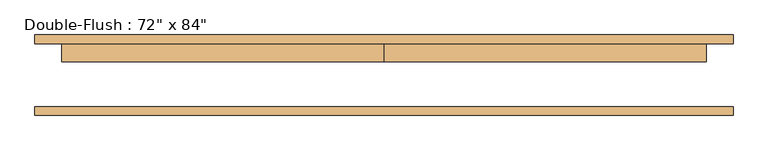
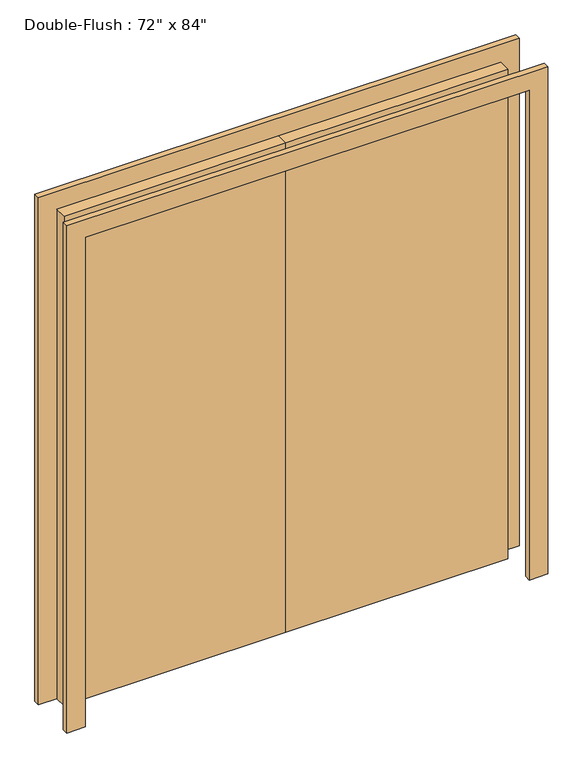
"""IFC4 building model written with IfcOpenShell, lengths in millimetres: door geometry."""

import ifcopenshell
import ifcopenshell.guid

model = None  # the IFC model being written
_history = None  # IfcOwnerHistory: only IFC2X3 demands one
_inside = {}  # id of a spatial element -> (the spatial element, [elements in it])
_under = {}  # id of a project, library or spatial element -> (it, [spatial elements below it])
_declared = {}  # id of a project -> (the project, [libraries it declares])
_typed = {}  # id of a type object -> (the type object, [elements of that type])
_made_of = {}  # id of a material, layer set ... -> (it, [elements and type objects made of it])


def new_model(schema):
    """Start an empty IFC model of exactly this schema.

    Asked for "IFC4X3", IfcOpenShell would pick the latest addendum, in which some entities
    have other attributes; the version numbers below select the first issue.
    IFC2X3 requires an IfcOwnerHistory on every rooted entity: one is made here for all.
    """
    global model, _history
    if schema == "IFC4X3":
        model = ifcopenshell.file(schema_version=(4, 3, 0, 0))
    else:
        model = ifcopenshell.file(schema=schema)
    _inside.clear()
    _under.clear()
    _declared.clear()
    _typed.clear()
    _made_of.clear()
    _history = None
    if model.schema == "IFC2X3":
        org = make("IfcOrganization", Name="unknown")
        user = make(
            "IfcPersonAndOrganization",
            ThePerson=make("IfcPerson", FamilyName="unknown"),
            TheOrganization=org,
        )
        app = make(
            "IfcApplication",
            ApplicationDeveloper=org,
            Version="unknown",
            ApplicationFullName="unknown",
            ApplicationIdentifier="unknown",
        )
        _history = make(
            "IfcOwnerHistory",
            OwningUser=user,
            OwningApplication=app,
            ChangeAction="ADDED",
            CreationDate=0,
        )
    return model


def make(cls, **values):
    """One entity of the class cls with the attributes given. An attribute that is None is left unset."""
    return model.create_entity(
        cls, **{name: value for name, value in values.items() if value is not None}
    )


def rooted(cls, **values):
    """An entity with a GlobalId (a new one), such as an element, a storey or a relation."""
    return make(cls, GlobalId=ifcopenshell.guid.new(), OwnerHistory=_history, **values)


def si_unit(unit_type, name, prefix=None):
    """IfcSIUnit, for example si_unit("LENGTHUNIT", "METRE", prefix="MILLI")."""
    return make("IfcSIUnit", UnitType=unit_type, Prefix=prefix, Name=name)


def assignment(units):
    """IfcUnitAssignment: the units of a project."""
    return None if units is None else make("IfcUnitAssignment", Units=units)


def point(xyz):
    """IfcCartesianPoint."""
    return None if xyz is None else make("IfcCartesianPoint", Coordinates=xyz)


def direction(xyz):
    """IfcDirection."""
    return None if xyz is None else make("IfcDirection", DirectionRatios=xyz)


def frame(location, z_axis=None, x_axis=None):
    """IfcAxis2Placement3D, a coordinate frame: its origin and axes. An axis left out is left unset."""
    return make(
        "IfcAxis2Placement3D",
        Location=point(location),
        Axis=direction(z_axis),
        RefDirection=direction(x_axis),
    )


def origin():
    """The frame at (0, 0, 0) with its axes left unset."""
    return frame((0.0, 0.0, 0.0))


def origin_with_axes():
    """The frame at (0, 0, 0) with the z axis (0, 0, 1) and the x axis (1, 0, 0) written out."""
    return frame((0.0, 0.0, 0.0), z_axis=(0.0, 0.0, 1.0), x_axis=(1.0, 0.0, 0.0))


def place(relative_to, where):
    """IfcLocalPlacement: puts the frame where relative to a parent placement (None: the world)."""
    return make(
        "IfcLocalPlacement", PlacementRelTo=relative_to, RelativePlacement=where
    )


def context(
    kind, dimensions, precision=None, world=None, true_north=None, identifier=None
):
    """IfcGeometricRepresentationContext, for example the 3D "Model" context."""
    return make(
        "IfcGeometricRepresentationContext",
        ContextIdentifier=identifier,
        ContextType=kind,
        CoordinateSpaceDimension=dimensions,
        Precision=precision,
        WorldCoordinateSystem=world,
        TrueNorth=true_north,
    )


def project(units=None, contexts=None):
    """IfcProject with its units and contexts."""
    return rooted(
        "IfcProject",
        Name="project",
        RepresentationContexts=contexts,
        UnitsInContext=assignment(units),
    )


def spatial(cls, under=None, at=None, **own):
    """A site, building, storey or space (cls), placed at a placement, below another one or the project."""
    s = rooted(cls, ObjectPlacement=at, **own)
    if under is not None:
        _under.setdefault(under.id(), (under, []))[1].append(s)
    return s


def polyline(points):
    """IfcPolyline through the points."""
    return make("IfcPolyline", Points=[point(p) for p in points])


def outline(outer, holes=None, kind="AREA"):
    """IfcArbitraryClosedProfileDef: a profile drawn as a closed curve; with holes, ...WithVoids."""
    if holes is None:
        return make("IfcArbitraryClosedProfileDef", ProfileType=kind, OuterCurve=outer)
    return make(
        "IfcArbitraryProfileDefWithVoids",
        ProfileType=kind,
        OuterCurve=outer,
        InnerCurves=holes,
    )


def extrude(swept, where, along, depth):
    """IfcExtrudedAreaSolid: the profile swept, set in the frame where, extruded along a direction by depth."""
    return make(
        "IfcExtrudedAreaSolid",
        SweptArea=swept,
        Position=where,
        ExtrudedDirection=direction(along),
        Depth=depth,
    )


def shape(context_of_items, identifier, shape_type, items):
    """IfcShapeRepresentation: the items that make up one representation, for example the "Body"."""
    return make(
        "IfcShapeRepresentation",
        ContextOfItems=context_of_items,
        RepresentationIdentifier=identifier,
        RepresentationType=shape_type,
        Items=items,
    )


def source(mapping_origin, context_of_items, identifier, shape_type, items):
    """IfcRepresentationMap: a shape defined once, which mapped items show again and again."""
    return make(
        "IfcRepresentationMap",
        MappingOrigin=mapping_origin,
        MappedRepresentation=shape(context_of_items, identifier, shape_type, items),
    )


def transform(
    local_origin,
    x_axis=None,
    y_axis=None,
    z_axis=None,
    scale=None,
    scale2=None,
    scale3=None,
    uniform=True,
):
    """IfcCartesianTransformationOperator3D, or its non-uniform kind. x_axis, y_axis, z_axis: its Axis1, 2, 3."""
    if uniform:
        return make(
            "IfcCartesianTransformationOperator3D",
            Axis1=direction(x_axis),
            Axis2=direction(y_axis),
            LocalOrigin=point(local_origin),
            Scale=scale,
            Axis3=direction(z_axis),
        )
    return make(
        "IfcCartesianTransformationOperator3DnonUniform",
        Axis1=direction(x_axis),
        Axis2=direction(y_axis),
        LocalOrigin=point(local_origin),
        Scale=scale,
        Axis3=direction(z_axis),
        Scale2=scale2,
        Scale3=scale3,
    )


def mapped(mapping_source, mapping_target):
    """IfcMappedItem: shows the shape of a source again, moved by a transform."""
    return make(
        "IfcMappedItem", MappingSource=mapping_source, MappingTarget=mapping_target
    )


def made_of(thing, what):
    """Note that an element or type object is made of a material, layer set ...; save() writes the relation."""
    if what is not None:
        _made_of.setdefault(what.id(), (what, []))[1].append(thing)
    return thing


def element(
    cls,
    number,
    at=None,
    inside=None,
    cuts=None,
    type_object=None,
    material=None,
    context=None,
    identifier="Body",
    shape_type=None,
    held_by="IfcProductDefinitionShape",
    body=None,
    shapes=None,
    **own,
):
    """One element of the class cls, such as IfcWall. Its Tag is "e" and its number.

    at: its placement. inside: the storey or other place that contains it. cuts: it is an
    opening in that element (IfcRelVoidsElement). A single representation is given by context,
    identifier, shape_type and body (its items); several are given by shapes. held_by: the class
    of the entity that holds the representations. save() writes the other relations.
    """
    e = rooted(cls, Tag="e%d" % number, ObjectPlacement=at, **own)
    if body is not None:
        shapes = [shape(context, identifier, shape_type, body)]
    if shapes is not None:
        e.Representation = make(held_by, Representations=shapes)
    if inside is not None:
        _inside.setdefault(inside.id(), (inside, []))[1].append(e)
    if cuts is not None:
        rooted(
            "IfcRelVoidsElement", RelatingBuildingElement=cuts, RelatedOpeningElement=e
        )
    if type_object is not None:
        _typed.setdefault(type_object.id(), (type_object, []))[1].append(e)
    return made_of(e, material)


def aggregate(whole, parts):
    """IfcRelAggregates: a whole, such as a stair, and the parts it consists of."""
    return rooted("IfcRelAggregates", RelatingObject=whole, RelatedObjects=parts)


def save(model, path):
    """Write the relations noted so far, then the file.

    IfcRelAggregates (storeys below a building ...), IfcRelContainedInSpatialStructure (elements
    in a storey), IfcRelDefinesByType, IfcRelAssociatesMaterial and IfcRelDeclares: one each for
    every whole, place, type object, material and project.
    """
    for whole, parts in _under.values():
        aggregate(whole, parts)
    for where, things in _inside.values():
        rooted(
            "IfcRelContainedInSpatialStructure",
            RelatedElements=things,
            RelatingStructure=where,
        )
    for kind, things in _typed.values():
        rooted("IfcRelDefinesByType", RelatedObjects=things, RelatingType=kind)
    for what, things in _made_of.values():
        rooted("IfcRelAssociatesMaterial", RelatedObjects=things, RelatingMaterial=what)
    for by, libraries in _declared.values():
        rooted("IfcRelDeclares", RelatingContext=by, RelatedDefinitions=libraries)
    model.write(path)


def door_798f09d1(model_context):
    return source(origin(), model_context, "Body", "SweptSolid", [
        extrude(outline(polyline([(0.0, 88.9), (914.4, 88.9), (914.4, 38.1), (0.0, 38.1), (0.0, 88.9)])), origin_with_axes(), (0.0, 0.0, 1.0), 2133.6),
        extrude(outline(polyline([(-914.4, 88.9), (0.0, 88.9), (0.0, 38.1), (-914.4, 38.1), (-914.4, 88.9)])), origin_with_axes(), (0.0, 0.0, 1.0), 2133.6),
        extrude(outline(polyline([(2133.6, -914.4), (2133.6, 914.4), (0.0, 914.4), (0.0, 990.6), (2209.8, 990.6), (2209.8, -990.6), (0.0, -990.6), (0.0, -914.4), (2133.6, -914.4)])), frame((0.0, -114.3, 0.0), z_axis=(0.0, 1.0, 0.0), x_axis=(0.0, 0.0, 1.0)), (0.0, 0.0, 1.0), 25.4),
        extrude(outline(polyline([(2133.6, -914.4), (2133.6, 914.4), (0.0, 914.4), (0.0, 990.6), (2209.8, 990.6), (2209.8, -990.6), (0.0, -990.6), (0.0, -914.4), (2133.6, -914.4)])), frame((0.0, 88.9, 0.0), z_axis=(0.0, 1.0, 0.0), x_axis=(0.0, 0.0, 1.0)), (0.0, 0.0, 1.0), 25.4),
    ])


if __name__ == "__main__":
    model = new_model("IFC4")
    model_context = context("Model", 3, world=origin())
    ifc_project = project(units=[si_unit("LENGTHUNIT", "METRE", prefix="MILLI")], contexts=[model_context])
    site = spatial("IfcSite", under=ifc_project)
    building = spatial("IfcBuilding", under=site)
    placement = place(None, origin())
    door_shape = door_798f09d1(model_context)
    element("IfcDoor", 1, ObjectType="Double-Flush : 72\" x 84\"", at=placement, inside=building, context=model_context, shape_type="MappedRepresentation", body=[
        mapped(door_shape, transform((0.0, 0.0, 0.0), x_axis=(1.0, 0.0, 0.0), y_axis=(0.0, 1.0, 0.0), z_axis=(0.0, 0.0, 1.0))),
    ])
    save(model, "model.ifc")

# Revit data of these elements
# Type "Double-Flush : 72\" x 84\""
#   Type Mark = "15"
#   Assembly Code = "C1020"
#   Thickness = 50.8 mm
#   Height = 2133.6 mm
#   Trim Projection Ext = 25.4 mm
#   Trim Projection Int = 25.4 mm
#   Trim Width = 76.2 mm
#   Width = 1828.8 mm
#   Door Material = Door - Panel
#   Frame Material = Door - Frame
#   Function = (empty or 0)
#   Wall Closure = (empty or 0)
# Element 1 (IfcDoor, "Double-Flush : 72\" x 84\"")
#   Materials on its faces: "Door - Frame", "Door - Panel"
# Materials
#   "Door - Panel": class "Wood", colour RGB 210 159 95, transparency 0
#   "Door - Frame": class "Miscellaneous", colour RGB 118 70 51, transparency 0
